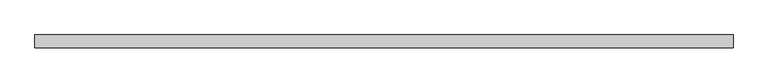
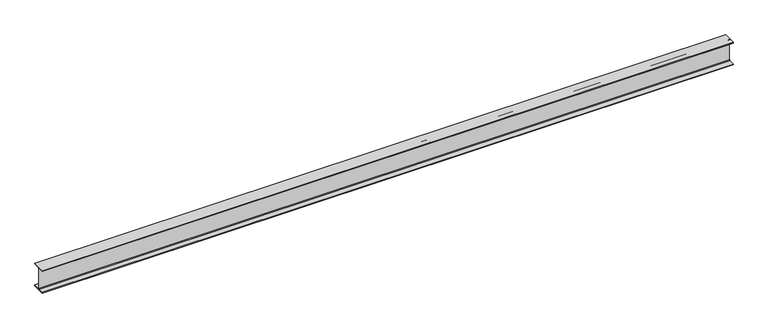
"""IFC4 building model written with IfcOpenShell, lengths in millimetres: beam geometry, Old_Steel Beam_H-KSD3502 : H_SB_ASB_H-390×300x10x16."""

from ifc_helpers import new_model, si_unit, point, frame, frame_2d, origin, place, context, project, spatial, polyline, circle_curve, trimmed, segment, composite_curve, outline, extrude, source, transform, mapped, element, save


def beam_513445db(model_context):
    return source(origin(), model_context, "Body", "SweptSolid", [
        extrude(outline(composite_curve([segment(polyline([(82.5, -141.5), (82.5, -151.7), (-82.5, -151.7), (-82.5, -141.5), (-11.9, -141.5)]), True, "CONTINUOUS"), segment(trimmed(circle_curve(frame_2d((-11.9, -132.6)), 8.9), [point((-11.9, -141.5))], [point((-3.0, -132.6))], True, "CARTESIAN"), True, "CONTINUOUS"), segment(polyline([(-3.0, -132.6), (-3.0, 132.6)]), True, "CONTINUOUS"), segment(trimmed(circle_curve(frame_2d((-11.9, 132.6)), 8.9), [point((-3.0, 132.6))], [point((-11.9, 141.5))], True, "CARTESIAN"), True, "CONTINUOUS"), segment(polyline([(-11.9, 141.5), (-82.5, 141.5), (-82.5, 151.7), (82.5, 151.7), (82.5, 141.5), (11.9, 141.5)]), True, "CONTINUOUS"), segment(trimmed(circle_curve(frame_2d((11.9, 132.6)), 8.9), [point((11.9, 141.5))], [point((3.0, 132.6))], True, "CARTESIAN"), True, "CONTINUOUS"), segment(polyline([(3.0, 132.6), (3.0, -132.6)]), True, "CONTINUOUS"), segment(trimmed(circle_curve(frame_2d((11.9, -132.6)), 8.9), [point((3.0, -132.6))], [point((11.9, -141.5))], True, "CARTESIAN"), True, "CONTINUOUS"), segment(polyline([(11.9, -141.5), (82.5, -141.5)]), True, "CONTINUOUS")], self_intersect=False)), frame((-4582.1993783, 0.0, 0.0), z_axis=(1.0, 0.0, 0.0), x_axis=(0.0, 1.0, 0.0)), (0.0, 0.0, 1.0), 8819.4993777),
    ])


if __name__ == "__main__":
    model = new_model("IFC4")
    model_context = context("Model", 3, world=origin())
    ifc_project = project(units=[si_unit("LENGTHUNIT", "METRE", prefix="MILLI")], contexts=[model_context])
    site = spatial("IfcSite", under=ifc_project)
    building = spatial("IfcBuilding", under=site)
    placement = place(None, origin())
    beam_shape = beam_513445db(model_context)
    element("IfcBeam", 1, ObjectType="Old_Steel Beam_H-KSD3502 : H_SB_ASB_H-390×300x10x16", at=placement, inside=building, context=model_context, shape_type="MappedRepresentation", body=[
        mapped(beam_shape, transform((0.0, 0.0, 0.0), x_axis=(1.0, 0.0, 0.0), y_axis=(0.0, 1.0, 0.0), z_axis=(0.0, 0.0, 1.0))),
    ])
    save(model, "model.ifc")

# Revit data of these elements
# Type "Old_Steel Beam_H-KSD3502 : H_SB_ASB_H-390×300x10x16"
#   Width = 30.0 cm
#   Web Thickness = 1.0 cm
#   Web Fillet = 2.2 cm
#   Warping Constant = 2517770.0 cm⁶
#   Torsional Moment of Inertia = 94.3867 cm⁴
#   Torsional Modulus = 1.0 cm³
#   Section Area = 136.0 cm²
#   Plastic Modulus weak axis = 733.0 cm³
#   Plastic Modulus strong axis = 2190.0 cm³
#   Perimeter = 1.92 m²/m
#   Nominal Weight = 107.00 kgf/m
#   Moment of Inertia weak axis = 7210.00 cm⁴
#   Moment of Inertia strong axis = 38700.00 cm⁴
#   Height = 39.0 cm
#   Flange Thickness = 1.6 cm
#   Elastic Modulus weak axis = 481.0 cm³
#   Elastic Modulus strong axis = 1980.0 cm³
#   Centroid Vertical = 19.5 cm
#   Centroid Horizontal = 15.0 cm
#   Length [instance default] = 1.5240 m
#   Structural Material [instance default] = Steel, 45-345
#   Assembly Code = ""
# Element 1 (IfcBeam, "Old_Steel Beam_H-KSD3502 : H_SB_ASB_H-390×300x10x16")
#   Structural Material = none
# Materials
#   "Steel, 45-345": class "Metal", colour RGB 189 187 185, transparency 0, Description = "Steel 345 MPa", Cost = 0
